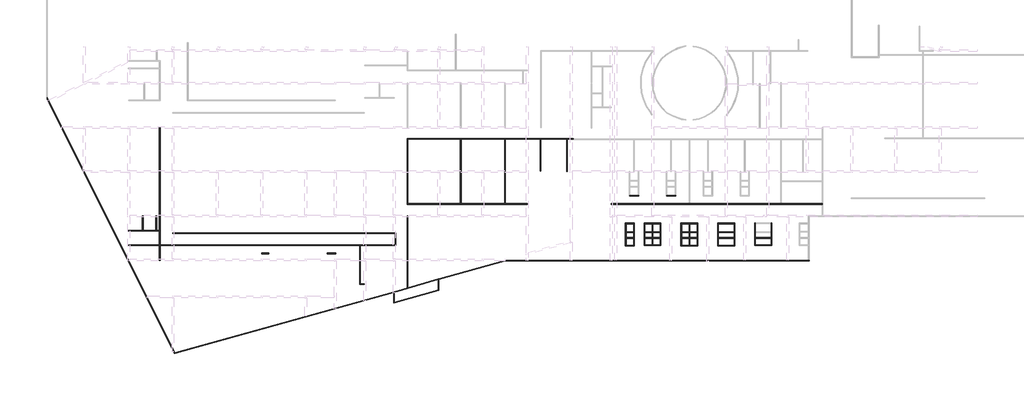
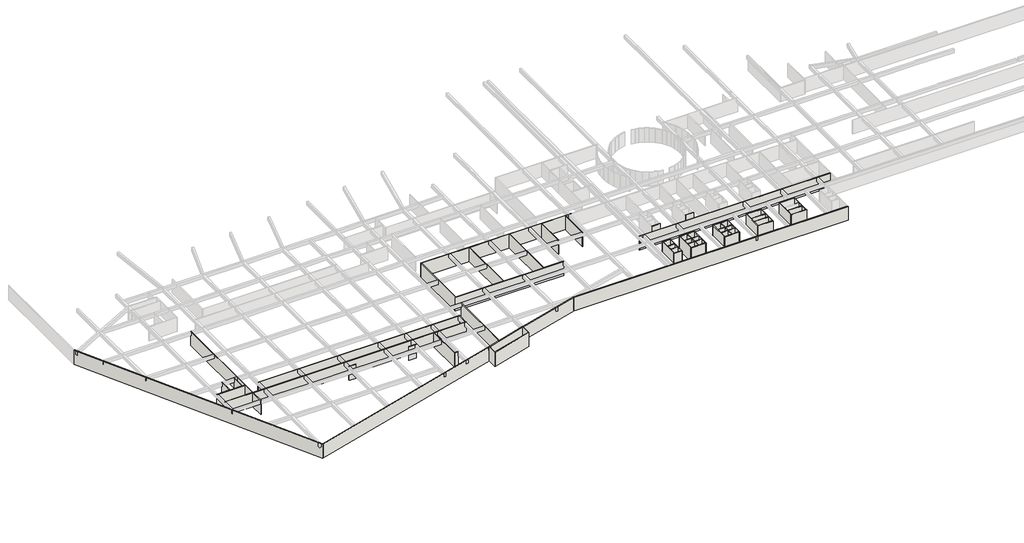
# One storey, part 1 of 8: 60 walls.
"""IFC4 building model written with IfcOpenShell, lengths in millimetres."""

from ifc_helpers import new_model, si_unit, origin, origin_with_axes, place, context, project, spatial, polyline, outline, extrude, faceted_brep, element, save

model = new_model("IFC4")

# Units and contexts
model_context = context("Model", 3, world=origin())
ifc_project = project(units=[si_unit("LENGTHUNIT", "METRE", prefix="MILLI")], contexts=[model_context])

# Site, building, storey
site = spatial("IfcSite", under=ifc_project)
building = spatial("IfcBuilding", under=site)
storey = spatial("IfcBuildingStorey", under=building, Name="户型图", Elevation=0.0)

# Walls
placement = place(None, origin())
element("IfcWall", 1, ObjectType="所有墙体", at=placement, inside=storey, context=model_context, shape_type="Brep", body=[
    faceted_brep([(299763.8653576, 3334.4623872, 0.0), (325653.4541666, -48444.7152378, 0.0), (325653.4541666, -48444.7152378, 3300.0), (299763.8653576, 3334.4623872, 3300.0), (299763.8653576, 3602.7905445, 0.0), (299763.8653576, 3602.7905445, 3300.0), (325716.5790893, -48302.6369258, 3300.0), (325771.2567723, -48411.9922918, 3300.0), (325771.2567723, -48411.9922918, 0.0), (325716.5790893, -48302.6369258, 0.0)], [[[0, 1, 2, 3]], [[4, 5, 6, 7, 8, 9]], [[1, 0, 4, 9, 8]], [[3, 2, 7, 6, 5]], [[0, 3, 5, 4]], [[2, 1, 8, 7]]]),
])
element("IfcWall", 2, ObjectType="所有墙体", at=placement, inside=storey, context=model_context, shape_type="Brep", body=[
    faceted_brep([(325771.2567723, -48411.9922918, 0.0), (370235.8958445, -36060.7036633, 0.0), (370355.8958445, -36027.37033, 0.0), (370355.8958445, -36027.37033, 3300.0), (370235.8958445, -36060.7036633, 3300.0), (325771.2567723, -48411.9922918, 3300.0), (325716.5790893, -48302.6369258, 0.0), (325716.5790893, -48302.6369258, 3300.0), (370355.8958445, -35902.8267187, 3300.0), (370355.8958445, -35902.8267187, 0.0), (370355.8958445, -36026.7458048, 0.0), (370355.8958445, -36026.7458048, 3300.0)], [[[0, 1, 2, 3, 4, 5]], [[6, 7, 8, 9]], [[2, 1, 0, 6, 9, 10]], [[5, 4, 3, 11, 8, 7]], [[0, 5, 7, 6]], [[3, 2, 10, 9, 8, 11]]]),
])
element("IfcWall", 3, ObjectType="所有墙体", at=placement, inside=storey, context=model_context, shape_type="Brep", body=[
    faceted_brep([(370235.8958445, -36060.7036633, 0.0), (370235.8958445, -38230.8455142, 0.0), (370235.8958445, -38230.8455142, 3300.0), (370235.8958445, -36060.7036633, 3300.0), (370355.8958445, -36027.37033, 0.0), (370355.8958445, -36027.37033, 3300.0), (370355.8958445, -38072.9685696, 3300.0), (370355.8958445, -38197.5121809, 3300.0), (370355.8958445, -38197.5121809, 0.0), (370355.8958445, -38072.9685696, 0.0)], [[[0, 1, 2, 3]], [[4, 5, 6, 7, 8, 9]], [[1, 0, 4, 9, 8]], [[3, 2, 7, 6, 5]], [[0, 3, 5, 4]], [[2, 1, 8, 7]]]),
])
element("IfcWall", 4, ObjectType="所有墙体", at=placement, inside=storey, context=model_context, shape_type="Brep", body=[
    faceted_brep([(370355.8958445, -38197.5121809, 0.0), (379412.9641952, -35681.6598618, 0.0), (379412.9641952, -35681.6598618, 3300.0), (370355.8958445, -38197.5121809, 3300.0), (370355.8958445, -38072.9685696, 0.0), (370355.8958445, -38072.9685696, 3300.0), (379292.9641952, -35590.4495838, 3300.0), (379412.9641952, -35557.1162505, 3300.0), (379412.9641952, -35557.1162505, 0.0), (379292.9641952, -35590.4495838, 0.0)], [[[0, 1, 2, 3]], [[4, 5, 6, 7, 8, 9]], [[1, 0, 4, 9, 8]], [[3, 2, 7, 6, 5]], [[0, 3, 5, 4]], [[2, 1, 8, 7]]]),
])
element("IfcWall", 5, ObjectType="所有墙体", at=placement, inside=storey, context=model_context, shape_type="Brep", body=[
    faceted_brep([(379412.9641952, -35557.1162505, 0.0), (379412.9641952, -33381.6598618, 0.0), (379412.9641952, -33257.1162505, 0.0), (379412.9641952, -33257.1162505, 3300.0), (379412.9641952, -33381.6598618, 3300.0), (379412.9641952, -35557.1162505, 3300.0), (379292.9641952, -35590.4495838, 0.0), (379292.9641952, -35590.4495838, 3300.0), (379292.9641952, -33416.0892021, 3300.0), (379292.9641952, -33291.074109, 3300.0), (379292.9641952, -33290.4495838, 3300.0), (379292.9641952, -33290.4495838, 0.0), (379292.9641952, -33291.074109, 0.0), (379292.9641952, -33416.0892021, 0.0)], [[[0, 1, 2, 3, 4, 5]], [[6, 7, 8, 9, 10, 11, 12, 13]], [[2, 1, 0, 6, 13, 12, 11]], [[5, 4, 3, 10, 9, 8, 7]], [[0, 5, 7, 6]], [[3, 2, 11, 10]]]),
])
element("IfcWall", 6, ObjectType="所有墙体", at=placement, inside=storey, context=model_context, shape_type="SweptSolid", body=[
    extrude(outline(polyline([(392926.9235644, -29627.78226), (379412.9641952, -33381.6598618), (379412.9641952, -33257.1162505), (392910.5665638, -29507.78226), (392926.9235644, -29627.78226)])), origin_with_axes(), (0.0, 0.0, 1.0), 3300.0),
])
element("IfcWall", 7, ObjectType="所有墙体", at=placement, inside=storey, context=model_context, shape_type="Brep", body=[
    faceted_brep([(392926.9235644, -29627.78226, 0.0), (454678.7450641, -29627.78226, 0.0), (454678.7450641, -29627.78226, 3300.0), (392926.9235644, -29627.78226, 3300.0), (392910.5665638, -29507.78226, 0.0), (392910.5665638, -29507.78226, 3300.0), (454558.7450641, -29507.78226, 3300.0), (454678.7450641, -29507.78226, 3300.0), (454678.7450641, -29507.78226, 0.0), (454558.7450641, -29507.78226, 0.0)], [[[0, 1, 2, 3]], [[4, 5, 6, 7, 8, 9]], [[1, 0, 4, 9, 8]], [[3, 2, 7, 6, 5]], [[0, 3, 5, 4]], [[2, 1, 8, 7]]]),
])
element("IfcWall", 8, ObjectType="所有墙体", at=placement, inside=storey, context=model_context, shape_type="Brep", body=[
    faceted_brep([(457393.8653576, -18001.3735105, 0.0), (449013.8653567, -18001.3735105, 0.0), (448893.8653567, -18001.3735105, 0.0), (430413.8653576, -18001.3735105, 0.0), (430293.8653576, -18001.3735105, 0.0), (414453.8653576, -18001.3735105, 0.0), (414453.8653576, -18001.3735105, 3300.0), (430293.8653576, -18001.3735105, 3300.0), (430413.8653576, -18001.3735105, 3300.0), (448893.8653567, -18001.3735105, 3300.0), (449013.8653567, -18001.3735105, 3300.0), (457393.8653576, -18001.3735105, 3300.0), (457393.8653576, -18121.3735105, 0.0), (457393.8653576, -18121.3735105, 3300.0), (414453.8653576, -18121.3735105, 3300.0), (414453.8653576, -18121.3735105, 0.0)], [[[0, 1, 2, 3, 4, 5, 6, 7, 8, 9, 10, 11]], [[12, 13, 14, 15]], [[5, 4, 3, 2, 1, 0, 12, 15]], [[6, 5, 15, 14]], [[11, 10, 9, 8, 7, 6, 14, 13]], [[0, 11, 13, 12]]]),
])
element("IfcWall", 9, ObjectType="所有墙体", at=placement, inside=storey, context=model_context, shape_type="Brep", body=[
    faceted_brep([(425763.8653576, -16421.3735096, 0.0), (427563.8653576, -16421.3735096, 0.0), (427563.8653576, -16421.3735096, 3300.0), (425763.8653576, -16421.3735096, 3300.0), (425763.8653576, -16301.3735096, 0.0), (425763.8653576, -16301.3735096, 3300.0), (427443.8653576, -16301.3735096, 3300.0), (427563.8653576, -16301.3735096, 3300.0), (427563.8653576, -16301.3735096, 0.0), (427443.8653576, -16301.3735096, 0.0)], [[[0, 1, 2, 3]], [[4, 5, 6, 7, 8, 9]], [[1, 0, 4, 9, 8]], [[3, 2, 7, 6, 5]], [[0, 3, 5, 4]], [[2, 1, 8, 7]]]),
])
element("IfcWall", 10, ObjectType="所有墙体", at=placement, inside=storey, context=model_context, shape_type="Brep", body=[
    faceted_brep([(418263.8653576, -16421.3261103, 0.0), (420063.8653576, -16421.3261103, 0.0), (420063.8653576, -16421.3261103, 3300.0), (418263.8653576, -16421.3261103, 3300.0), (418263.8653576, -16301.3261103, 0.0), (418263.8653576, -16301.3261103, 3300.0), (419943.8653576, -16301.3261103, 3300.0), (420063.8653576, -16301.3261103, 3300.0), (420063.8653576, -16301.3261103, 0.0), (419943.8653576, -16301.3261103, 0.0)], [[[0, 1, 2, 3]], [[4, 5, 6, 7, 8, 9]], [[1, 0, 4, 9, 8]], [[3, 2, 7, 6, 5]], [[0, 3, 5, 4]], [[2, 1, 8, 7]]]),
])
element("IfcWall", 11, ObjectType="所有墙体", at=placement, inside=storey, context=model_context, shape_type="Brep", body=[
    faceted_brep([(417343.8653576, -22071.3735096, 0.0), (417463.8653576, -22071.3735096, 0.0), (419043.8653576, -22071.3735096, 0.0), (419163.8653576, -22071.3735096, 0.0), (419163.8653576, -22071.3735096, 3300.0), (419043.8653576, -22071.3735096, 3300.0), (417463.8653576, -22071.3735096, 3300.0), (417343.8653576, -22071.3735096, 3300.0), (417343.8653576, -21951.3735096, 0.0), (417343.8653576, -21951.3735096, 3300.0), (419163.8653576, -21951.3735096, 3300.0), (419163.8653576, -21951.3735096, 0.0)], [[[0, 1, 2, 3, 4, 5, 6, 7]], [[8, 9, 10, 11]], [[3, 2, 1, 0, 8, 11]], [[7, 6, 5, 4, 10, 9]], [[4, 3, 11, 10]], [[0, 7, 9, 8]]]),
])
element("IfcWall", 12, ObjectType="所有墙体", at=placement, inside=storey, context=model_context, shape_type="Brep", body=[
    faceted_brep([(419043.8653576, -22071.3735096, 0.0), (419043.8653576, -23701.6182553, 0.0), (419043.8653576, -23821.6182553, 0.0), (419043.8653576, -24901.6891861, 0.0), (419043.8653576, -25021.6891861, 0.0), (419043.8653576, -26451.3735096, 0.0), (419043.8653576, -26571.3735096, 0.0), (419043.8653576, -26571.3735096, 3300.0), (419043.8653576, -26451.3735096, 3300.0), (419043.8653576, -25021.6891861, 3300.0), (419043.8653576, -24901.6891861, 3300.0), (419043.8653576, -23821.6182553, 3300.0), (419043.8653576, -23701.6182553, 3300.0), (419043.8653576, -22071.3735096, 3300.0), (419163.8653576, -22071.3735096, 0.0), (419163.8653576, -22071.3735096, 3300.0), (419163.8653576, -26571.3735096, 3300.0), (419163.8653576, -26571.3735096, 0.0)], [[[0, 1, 2, 3, 4, 5, 6, 7, 8, 9, 10, 11, 12, 13]], [[14, 15, 16, 17]], [[6, 5, 4, 3, 2, 1, 0, 14, 17]], [[13, 12, 11, 10, 9, 8, 7, 16, 15]], [[0, 13, 15, 14]], [[7, 6, 17, 16]]]),
])
element("IfcWall", 13, ObjectType="所有墙体", at=placement, inside=storey, context=model_context, shape_type="Brep", body=[
    faceted_brep([(419043.8653576, -26451.3735096, 0.0), (417463.8653576, -26451.3735096, 0.0), (417343.8653576, -26451.3735096, 0.0), (417343.8653576, -26451.3735096, 3300.0), (417463.8653576, -26451.3735096, 3300.0), (419043.8653576, -26451.3735096, 3300.0), (419043.8653576, -26571.3735096, 0.0), (419043.8653576, -26571.3735096, 3300.0), (417343.8653576, -26571.3735096, 3300.0), (417343.8653576, -26571.3735096, 0.0)], [[[0, 1, 2, 3, 4, 5]], [[6, 7, 8, 9]], [[2, 1, 0, 6, 9]], [[5, 4, 3, 8, 7]], [[0, 5, 7, 6]], [[3, 2, 9, 8]]]),
])
element("IfcWall", 14, ObjectType="所有墙体", at=placement, inside=storey, context=model_context, shape_type="Brep", body=[
    faceted_brep([(417463.8653576, -26451.3735096, 0.0), (417463.8653576, -25021.6891861, 0.0), (417463.8653576, -24901.6891861, 0.0), (417463.8653576, -23821.6182553, 0.0), (417463.8653576, -23701.6182553, 0.0), (417463.8653576, -22071.3735096, 0.0), (417463.8653576, -22071.3735096, 3300.0), (417463.8653576, -23701.6182553, 3300.0), (417463.8653576, -23821.6182553, 3300.0), (417463.8653576, -24901.6891861, 3300.0), (417463.8653576, -25021.6891861, 3300.0), (417463.8653576, -26451.3735096, 3300.0), (417343.8653576, -26451.3735096, 0.0), (417343.8653576, -26451.3735096, 3300.0), (417343.8653576, -22071.3735096, 3300.0), (417343.8653576, -22071.3735096, 0.0)], [[[0, 1, 2, 3, 4, 5, 6, 7, 8, 9, 10, 11]], [[12, 13, 14, 15]], [[5, 4, 3, 2, 1, 0, 12, 15]], [[11, 10, 9, 8, 7, 6, 14, 13]], [[6, 5, 15, 14]], [[0, 11, 13, 12]]]),
])
element("IfcWall", 15, ObjectType="所有墙体", at=placement, inside=storey, context=model_context, shape_type="SweptSolid", body=[
    extrude(outline(polyline([(417463.8653576, -23701.6182553), (419043.8653576, -23701.6182553), (419043.8653576, -23821.6182553), (417463.8653576, -23821.6182553), (417463.8653576, -23701.6182553)])), origin_with_axes(), (0.0, 0.0, 1.0), 3300.0),
])
element("IfcWall", 16, ObjectType="所有墙体", at=placement, inside=storey, context=model_context, shape_type="SweptSolid", body=[
    extrude(outline(polyline([(419043.8653576, -25021.6891861), (417463.8653576, -25021.6891861), (417463.8653576, -24901.6891861), (419043.8653576, -24901.6891861), (419043.8653576, -25021.6891861)])), origin_with_axes(), (0.0, 0.0, 1.0), 3300.0),
])
element("IfcWall", 17, ObjectType="所有墙体", at=placement, inside=storey, context=model_context, shape_type="Brep", body=[
    faceted_brep([(421144.3420584, -22071.3735096, 0.0), (421264.3420584, -22071.3735096, 0.0), (422793.8653536, -22071.3735096, 0.0), (422913.8653536, -22071.3735096, 0.0), (424443.3886489, -22071.3735096, 0.0), (424563.3886489, -22071.3735096, 0.0), (424563.3886489, -22071.3735096, 3300.0), (424443.3886489, -22071.3735096, 3300.0), (422913.8653536, -22071.3735096, 3300.0), (422793.8653536, -22071.3735096, 3300.0), (421264.3420584, -22071.3735096, 3300.0), (421144.3420584, -22071.3735096, 3300.0), (421144.3420584, -21951.3735096, 0.0), (421144.3420584, -21951.3735096, 3300.0), (424563.3886489, -21951.3735096, 3300.0), (424563.3886489, -21951.3735096, 0.0)], [[[0, 1, 2, 3, 4, 5, 6, 7, 8, 9, 10, 11]], [[12, 13, 14, 15]], [[5, 4, 3, 2, 1, 0, 12, 15]], [[11, 10, 9, 8, 7, 6, 14, 13]], [[6, 5, 15, 14]], [[0, 11, 13, 12]]]),
])
element("IfcWall", 18, ObjectType="所有墙体", at=placement, inside=storey, context=model_context, shape_type="Brep", body=[
    faceted_brep([(424443.3886489, -22071.3735096, 0.0), (424443.3886489, -23701.6182553, 0.0), (424443.3886489, -23821.6182553, 0.0), (424443.3886489, -24901.6891861, 0.0), (424443.3886489, -25021.6891861, 0.0), (424443.3886489, -26401.6891861, 0.0), (424443.3886489, -26521.6891861, 0.0), (424443.3886489, -26521.6891861, 3300.0), (424443.3886489, -26401.6891861, 3300.0), (424443.3886489, -25021.6891861, 3300.0), (424443.3886489, -24901.6891861, 3300.0), (424443.3886489, -23821.6182553, 3300.0), (424443.3886489, -23701.6182553, 3300.0), (424443.3886489, -22071.3735096, 3300.0), (424563.3886489, -22071.3735096, 0.0), (424563.3886489, -22071.3735096, 3300.0), (424563.3886489, -26521.6891861, 3300.0), (424563.3886489, -26521.6891861, 0.0)], [[[0, 1, 2, 3, 4, 5, 6, 7, 8, 9, 10, 11, 12, 13]], [[14, 15, 16, 17]], [[6, 5, 4, 3, 2, 1, 0, 14, 17]], [[13, 12, 11, 10, 9, 8, 7, 16, 15]], [[0, 13, 15, 14]], [[7, 6, 17, 16]]]),
])
element("IfcWall", 19, ObjectType="所有墙体", at=placement, inside=storey, context=model_context, shape_type="Brep", body=[
    faceted_brep([(424443.3886489, -26401.6891861, 0.0), (422913.8653536, -26401.6891861, 0.0), (422793.8653536, -26401.6891861, 0.0), (421264.3420584, -26401.6891861, 0.0), (421144.3420584, -26401.6891861, 0.0), (421144.3420584, -26401.6891861, 3300.0), (421264.3420584, -26401.6891861, 3300.0), (422793.8653536, -26401.6891861, 3300.0), (422913.8653536, -26401.6891861, 3300.0), (424443.3886489, -26401.6891861, 3300.0), (424443.3886489, -26521.6891861, 0.0), (424443.3886489, -26521.6891861, 3300.0), (421144.3420584, -26521.6891861, 3300.0), (421144.3420584, -26521.6891861, 0.0)], [[[0, 1, 2, 3, 4, 5, 6, 7, 8, 9]], [[10, 11, 12, 13]], [[4, 3, 2, 1, 0, 10, 13]], [[9, 8, 7, 6, 5, 12, 11]], [[0, 9, 11, 10]], [[5, 4, 13, 12]]]),
])
element("IfcWall", 20, ObjectType="所有墙体", at=placement, inside=storey, context=model_context, shape_type="Brep", body=[
    faceted_brep([(421264.3420584, -26401.6891861, 0.0), (421264.3420584, -25021.6891861, 0.0), (421264.3420584, -24901.6891861, 0.0), (421264.3420584, -23821.6182553, 0.0), (421264.3420584, -23701.6182553, 0.0), (421264.3420584, -22071.3735096, 0.0), (421264.3420584, -22071.3735096, 3300.0), (421264.3420584, -23701.6182553, 3300.0), (421264.3420584, -23821.6182553, 3300.0), (421264.3420584, -24901.6891861, 3300.0), (421264.3420584, -25021.6891861, 3300.0), (421264.3420584, -26401.6891861, 3300.0), (421144.3420584, -26401.6891861, 0.0), (421144.3420584, -26401.6891861, 3300.0), (421144.3420584, -22071.3735096, 3300.0), (421144.3420584, -22071.3735096, 0.0)], [[[0, 1, 2, 3, 4, 5, 6, 7, 8, 9, 10, 11]], [[12, 13, 14, 15]], [[5, 4, 3, 2, 1, 0, 12, 15]], [[11, 10, 9, 8, 7, 6, 14, 13]], [[0, 11, 13, 12]], [[6, 5, 15, 14]]]),
])
element("IfcWall", 21, ObjectType="所有墙体", at=placement, inside=storey, context=model_context, shape_type="Brep", body=[
    faceted_brep([(422793.8653536, -22071.3735096, 0.0), (422793.8653536, -23701.6182553, 0.0), (422793.8653536, -23821.6182553, 0.0), (422793.8653536, -24901.6891861, 0.0), (422793.8653536, -25021.6891861, 0.0), (422793.8653536, -26401.6891861, 0.0), (422793.8653536, -26401.6891861, 3300.0), (422793.8653536, -25021.6891861, 3300.0), (422793.8653536, -24901.6891861, 3300.0), (422793.8653536, -23821.6182553, 3300.0), (422793.8653536, -23701.6182553, 3300.0), (422793.8653536, -22071.3735096, 3300.0), (422913.8653536, -22071.3735096, 0.0), (422913.8653536, -22071.3735096, 3300.0), (422913.8653536, -23701.6182553, 3300.0), (422913.8653536, -23821.6182553, 3300.0), (422913.8653536, -24901.6891861, 3300.0), (422913.8653536, -25021.6891861, 3300.0), (422913.8653536, -26401.6891861, 3300.0), (422913.8653536, -26401.6891861, 0.0), (422913.8653536, -25021.6891861, 0.0), (422913.8653536, -24901.6891861, 0.0), (422913.8653536, -23821.6182553, 0.0), (422913.8653536, -23701.6182553, 0.0)], [[[0, 1, 2, 3, 4, 5, 6, 7, 8, 9, 10, 11]], [[12, 13, 14, 15, 16, 17, 18, 19, 20, 21, 22, 23]], [[5, 4, 3, 2, 1, 0, 12, 23, 22, 21, 20, 19]], [[11, 10, 9, 8, 7, 6, 18, 17, 16, 15, 14, 13]], [[0, 11, 13, 12]], [[6, 5, 19, 18]]]),
])
element("IfcWall", 22, ObjectType="所有墙体", at=placement, inside=storey, context=model_context, shape_type="SweptSolid", body=[
    extrude(outline(polyline([(424443.3886489, -23701.6182553), (424443.3886489, -23821.6182553), (422913.8653536, -23821.6182553), (422913.8653536, -23701.6182553), (424443.3886489, -23701.6182553)])), origin_with_axes(), (0.0, 0.0, 1.0), 3300.0),
    extrude(outline(polyline([(421264.3420584, -23821.6182553), (421264.3420584, -23701.6182553), (422793.8653536, -23701.6182553), (422793.8653536, -23821.6182553), (421264.3420584, -23821.6182553)])), origin_with_axes(), (0.0, 0.0, 1.0), 3300.0),
])
element("IfcWall", 23, ObjectType="所有墙体", at=placement, inside=storey, context=model_context, shape_type="SweptSolid", body=[
    extrude(outline(polyline([(424443.3886489, -24901.6891861), (424443.3886489, -25021.6891861), (422913.8653536, -25021.6891861), (422913.8653536, -24901.6891861), (424443.3886489, -24901.6891861)])), origin_with_axes(), (0.0, 0.0, 1.0), 3300.0),
    extrude(outline(polyline([(421264.3420584, -25021.6891861), (421264.3420584, -24901.6891861), (422793.8653536, -24901.6891861), (422793.8653536, -25021.6891861), (421264.3420584, -25021.6891861)])), origin_with_axes(), (0.0, 0.0, 1.0), 3300.0),
])
element("IfcWall", 24, ObjectType="所有墙体", at=placement, inside=storey, context=model_context, shape_type="Brep", body=[
    faceted_brep([(428643.3886489, -22071.3735096, 0.0), (428763.3886489, -22071.3735096, 0.0), (430293.3886489, -22071.3735096, 0.0), (430413.3886489, -22071.3735096, 0.0), (431943.3886489, -22071.3735096, 0.0), (432063.3886489, -22071.3735096, 0.0), (432063.3886489, -22071.3735096, 3300.0), (431943.3886489, -22071.3735096, 3300.0), (430413.3886489, -22071.3735096, 3300.0), (430293.3886489, -22071.3735096, 3300.0), (428763.3886489, -22071.3735096, 3300.0), (428643.3886489, -22071.3735096, 3300.0), (428643.3886489, -21951.3735096, 0.0), (428643.3886489, -21951.3735096, 3300.0), (432063.3886489, -21951.3735096, 3300.0), (432063.3886489, -21951.3735096, 0.0)], [[[0, 1, 2, 3, 4, 5, 6, 7, 8, 9, 10, 11]], [[12, 13, 14, 15]], [[5, 4, 3, 2, 1, 0, 12, 15]], [[11, 10, 9, 8, 7, 6, 14, 13]], [[6, 5, 15, 14]], [[0, 11, 13, 12]]]),
])
element("IfcWall", 25, ObjectType="所有墙体", at=placement, inside=storey, context=model_context, shape_type="Brep", body=[
    faceted_brep([(431943.3886489, -22071.3735096, 0.0), (431943.3886489, -23701.6182553, 0.0), (431943.3886489, -23821.6182553, 0.0), (431943.3886489, -24901.6891861, 0.0), (431943.3886489, -25021.6891861, 0.0), (431943.3886489, -26451.6891861, 0.0), (431943.3886489, -26571.6891861, 0.0), (431943.3886489, -26571.6891861, 3300.0), (431943.3886489, -26451.6891861, 3300.0), (431943.3886489, -25021.6891861, 3300.0), (431943.3886489, -24901.6891861, 3300.0), (431943.3886489, -23821.6182553, 3300.0), (431943.3886489, -23701.6182553, 3300.0), (431943.3886489, -22071.3735096, 3300.0), (432063.3886489, -22071.3735096, 0.0), (432063.3886489, -22071.3735096, 3300.0), (432063.3886489, -26571.6891861, 3300.0), (432063.3886489, -26571.6891861, 0.0)], [[[0, 1, 2, 3, 4, 5, 6, 7, 8, 9, 10, 11, 12, 13]], [[14, 15, 16, 17]], [[6, 5, 4, 3, 2, 1, 0, 14, 17]], [[13, 12, 11, 10, 9, 8, 7, 16, 15]], [[0, 13, 15, 14]], [[7, 6, 17, 16]]]),
])
element("IfcWall", 26, ObjectType="所有墙体", at=placement, inside=storey, context=model_context, shape_type="Brep", body=[
    faceted_brep([(431943.3886489, -26451.6891861, 0.0), (430413.3886489, -26451.6891861, 0.0), (430293.3886489, -26451.6891861, 0.0), (428763.3886489, -26451.6891861, 0.0), (428643.3886489, -26451.6891861, 0.0), (428643.3886489, -26451.6891861, 3300.0), (428763.3886489, -26451.6891861, 3300.0), (430293.3886489, -26451.6891861, 3300.0), (430413.3886489, -26451.6891861, 3300.0), (431943.3886489, -26451.6891861, 3300.0), (431943.3886489, -26571.6891861, 0.0), (431943.3886489, -26571.6891861, 3300.0), (428643.3886489, -26571.6891861, 3300.0), (428643.3886489, -26571.6891861, 0.0)], [[[0, 1, 2, 3, 4, 5, 6, 7, 8, 9]], [[10, 11, 12, 13]], [[4, 3, 2, 1, 0, 10, 13]], [[9, 8, 7, 6, 5, 12, 11]], [[0, 9, 11, 10]], [[5, 4, 13, 12]]]),
])
element("IfcWall", 27, ObjectType="所有墙体", at=placement, inside=storey, context=model_context, shape_type="Brep", body=[
    faceted_brep([(428763.3886489, -26451.6891861, 0.0), (428763.3886489, -25021.6891861, 0.0), (428763.3886489, -24901.6891861, 0.0), (428763.3886489, -23821.6182553, 0.0), (428763.3886489, -23701.6182553, 0.0), (428763.3886489, -22071.3735096, 0.0), (428763.3886489, -22071.3735096, 3300.0), (428763.3886489, -23701.6182553, 3300.0), (428763.3886489, -23821.6182553, 3300.0), (428763.3886489, -24901.6891861, 3300.0), (428763.3886489, -25021.6891861, 3300.0), (428763.3886489, -26451.6891861, 3300.0), (428643.3886489, -26451.6891861, 0.0), (428643.3886489, -26451.6891861, 3300.0), (428643.3886489, -22071.3735096, 3300.0), (428643.3886489, -22071.3735096, 0.0)], [[[0, 1, 2, 3, 4, 5, 6, 7, 8, 9, 10, 11]], [[12, 13, 14, 15]], [[5, 4, 3, 2, 1, 0, 12, 15]], [[11, 10, 9, 8, 7, 6, 14, 13]], [[6, 5, 15, 14]], [[0, 11, 13, 12]]]),
])
element("IfcWall", 28, ObjectType="所有墙体", at=placement, inside=storey, context=model_context, shape_type="Brep", body=[
    faceted_brep([(428763.3886489, -23821.6182553, 0.0), (430293.3886489, -23821.6182553, 0.0), (430413.3886489, -23821.6182553, 0.0), (431943.3886489, -23821.6182553, 0.0), (431943.3886489, -23821.6182553, 3300.0), (430413.3886489, -23821.6182553, 3300.0), (430293.3886489, -23821.6182553, 3300.0), (428763.3886489, -23821.6182553, 3300.0), (428763.3886489, -23701.6182553, 0.0), (428763.3886489, -23701.6182553, 3300.0), (430293.3886489, -23701.6182553, 3300.0), (430413.3886489, -23701.6182553, 3300.0), (431943.3886489, -23701.6182553, 3300.0), (431943.3886489, -23701.6182553, 0.0), (430413.3886489, -23701.6182553, 0.0), (430293.3886489, -23701.6182553, 0.0)], [[[0, 1, 2, 3, 4, 5, 6, 7]], [[8, 9, 10, 11, 12, 13, 14, 15]], [[3, 2, 1, 0, 8, 15, 14, 13]], [[7, 6, 5, 4, 12, 11, 10, 9]], [[4, 3, 13, 12]], [[0, 7, 9, 8]]]),
])
element("IfcWall", 29, ObjectType="所有墙体", at=placement, inside=storey, context=model_context, shape_type="Brep", body=[
    faceted_brep([(431943.3886489, -24901.6891861, 0.0), (430413.3886489, -24901.6891861, 0.0), (430293.3886489, -24901.6891861, 0.0), (428763.3886489, -24901.6891861, 0.0), (428763.3886489, -24901.6891861, 3300.0), (430293.3886489, -24901.6891861, 3300.0), (430413.3886489, -24901.6891861, 3300.0), (431943.3886489, -24901.6891861, 3300.0), (431943.3886489, -25021.6891861, 0.0), (431943.3886489, -25021.6891861, 3300.0), (430413.3886489, -25021.6891861, 3300.0), (430293.3886489, -25021.6891861, 3300.0), (428763.3886489, -25021.6891861, 3300.0), (428763.3886489, -25021.6891861, 0.0), (430293.3886489, -25021.6891861, 0.0), (430413.3886489, -25021.6891861, 0.0)], [[[0, 1, 2, 3, 4, 5, 6, 7]], [[8, 9, 10, 11, 12, 13, 14, 15]], [[3, 2, 1, 0, 8, 15, 14, 13]], [[7, 6, 5, 4, 12, 11, 10, 9]], [[0, 7, 9, 8]], [[4, 3, 13, 12]]]),
])
element("IfcWall", 30, ObjectType="所有墙体", at=placement, inside=storey, context=model_context, shape_type="SweptSolid", body=[
    extrude(outline(polyline([(430293.3886489, -22071.3735096), (430413.3886489, -22071.3735096), (430413.3886489, -23701.6182553), (430293.3886489, -23701.6182553), (430293.3886489, -22071.3735096)])), origin_with_axes(), (0.0, 0.0, 1.0), 3300.0),
    extrude(outline(polyline([(430413.3886489, -26451.6891861), (430293.3886489, -26451.6891861), (430293.3886489, -25021.6891861), (430413.3886489, -25021.6891861), (430413.3886489, -26451.6891861)])), origin_with_axes(), (0.0, 0.0, 1.0), 3300.0),
    extrude(outline(polyline([(430293.3886489, -23821.6182553), (430413.3886489, -23821.6182553), (430413.3886489, -24901.6891861), (430293.3886489, -24901.6891861), (430293.3886489, -23821.6182553)])), origin_with_axes(), (0.0, 0.0, 1.0), 3300.0),
])
element("IfcWall", 31, ObjectType="所有墙体", at=placement, inside=storey, context=model_context, shape_type="Brep", body=[
    faceted_brep([(436144.3420663, -21951.6891861, 0.0), (436144.3420663, -26571.6891861, 0.0), (436144.3420663, -26571.6891861, 3300.0), (436144.3420663, -21951.6891861, 3300.0), (436264.3420663, -21951.6891861, 0.0), (436264.3420663, -21951.6891861, 3300.0), (436264.3420663, -22071.6891861, 3300.0), (436264.3420663, -23701.6182553, 3300.0), (436264.3420663, -23821.6182553, 3300.0), (436264.3420663, -24901.6891861, 3300.0), (436264.3420663, -25021.6891861, 3300.0), (436264.3420663, -26451.6891861, 3300.0), (436264.3420663, -26571.6891861, 3300.0), (436264.3420663, -26571.6891861, 0.0), (436264.3420663, -26451.6891861, 0.0), (436264.3420663, -25021.6891861, 0.0), (436264.3420663, -24901.6891861, 0.0), (436264.3420663, -23821.6182553, 0.0), (436264.3420663, -23701.6182553, 0.0), (436264.3420663, -22071.6891861, 0.0)], [[[0, 1, 2, 3]], [[4, 5, 6, 7, 8, 9, 10, 11, 12, 13, 14, 15, 16, 17, 18, 19]], [[1, 0, 4, 19, 18, 17, 16, 15, 14, 13]], [[3, 2, 12, 11, 10, 9, 8, 7, 6, 5]], [[2, 1, 13, 12]], [[0, 3, 5, 4]]]),
])
element("IfcWall", 32, ObjectType="所有墙体", at=placement, inside=storey, context=model_context, shape_type="Brep", body=[
    faceted_brep([(436264.3420663, -26571.6891861, 0.0), (439564.3420663, -26571.6891861, 0.0), (439564.3420663, -26571.6891861, 3300.0), (436264.3420663, -26571.6891861, 3300.0), (436264.3420663, -26451.6891861, 0.0), (436264.3420663, -26451.6891861, 3300.0), (439444.3420663, -26451.6891861, 3300.0), (439564.3420663, -26451.6891861, 3300.0), (439564.3420663, -26451.6891861, 0.0), (439444.3420663, -26451.6891861, 0.0)], [[[0, 1, 2, 3]], [[4, 5, 6, 7, 8, 9]], [[1, 0, 4, 9, 8]], [[3, 2, 7, 6, 5]], [[0, 3, 5, 4]], [[2, 1, 8, 7]]]),
])
element("IfcWall", 33, ObjectType="所有墙体", at=placement, inside=storey, context=model_context, shape_type="Brep", body=[
    faceted_brep([(439564.3420663, -26451.6891861, 0.0), (439564.3420663, -21951.6891861, 0.0), (439564.3420663, -21951.6891861, 3300.0), (439564.3420663, -26451.6891861, 3300.0), (439444.3420663, -26451.6891861, 0.0), (439444.3420663, -26451.6891861, 3300.0), (439444.3420663, -25021.6891861, 3300.0), (439444.3420663, -24901.6891861, 3300.0), (439444.3420663, -23821.6182553, 3300.0), (439444.3420663, -23701.6182553, 3300.0), (439444.3420663, -22071.6891861, 3300.0), (439444.3420663, -21951.6891861, 3300.0), (439444.3420663, -21951.6891861, 0.0), (439444.3420663, -22071.6891861, 0.0), (439444.3420663, -23701.6182553, 0.0), (439444.3420663, -23821.6182553, 0.0), (439444.3420663, -24901.6891861, 0.0), (439444.3420663, -25021.6891861, 0.0)], [[[0, 1, 2, 3]], [[4, 5, 6, 7, 8, 9, 10, 11, 12, 13, 14, 15, 16, 17]], [[1, 0, 4, 17, 16, 15, 14, 13, 12]], [[3, 2, 11, 10, 9, 8, 7, 6, 5]], [[0, 3, 5, 4]], [[2, 1, 12, 11]]]),
])
element("IfcWall", 34, ObjectType="所有墙体", at=placement, inside=storey, context=model_context, shape_type="SweptSolid", body=[
    extrude(outline(polyline([(436264.3420663, -21951.6891861), (439444.3420663, -21951.6891861), (439444.3420663, -22071.6891861), (436264.3420663, -22071.6891861), (436264.3420663, -21951.6891861)])), origin_with_axes(), (0.0, 0.0, 1.0), 3300.0),
])
element("IfcWall", 35, ObjectType="所有墙体", at=placement, inside=storey, context=model_context, shape_type="SweptSolid", body=[
    extrude(outline(polyline([(439444.3420663, -23821.6182553), (436264.3420663, -23821.6182553), (436264.3420663, -23701.6182553), (439444.3420663, -23701.6182553), (439444.3420663, -23821.6182553)])), origin_with_axes(), (0.0, 0.0, 1.0), 3300.0),
])
element("IfcWall", 36, ObjectType="所有墙体", at=placement, inside=storey, context=model_context, shape_type="SweptSolid", body=[
    extrude(outline(polyline([(436264.3420663, -24901.6891861), (439444.3420663, -24901.6891861), (439444.3420663, -25021.6891861), (436264.3420663, -25021.6891861), (436264.3420663, -24901.6891861)])), origin_with_axes(), (0.0, 0.0, 1.0), 3300.0),
])
element("IfcWall", 37, ObjectType="所有墙体", at=placement, inside=storey, context=model_context, shape_type="Brep", body=[
    faceted_brep([(443593.8653655, -21921.3735096, 0.0), (443593.8653655, -26521.3735096, 0.0), (443593.8653655, -26521.3735096, 3300.0), (443593.8653655, -21921.3735096, 3300.0), (443713.8653655, -21921.3735096, 0.0), (443713.8653655, -21921.3735096, 3300.0), (443713.8653655, -22041.3735096, 3300.0), (443713.8653655, -23701.6182553, 3300.0), (443713.8653655, -23821.6182553, 3300.0), (443713.8653655, -24901.6891611, 3300.0), (443713.8653655, -25021.6891611, 3300.0), (443713.8653655, -26401.3735096, 3300.0), (443713.8653655, -26521.3735096, 3300.0), (443713.8653655, -26521.3735096, 0.0), (443713.8653655, -26401.3735096, 0.0), (443713.8653655, -25021.6891611, 0.0), (443713.8653655, -24901.6891611, 0.0), (443713.8653655, -23821.6182553, 0.0), (443713.8653655, -23701.6182553, 0.0), (443713.8653655, -22041.3735096, 0.0)], [[[0, 1, 2, 3]], [[4, 5, 6, 7, 8, 9, 10, 11, 12, 13, 14, 15, 16, 17, 18, 19]], [[1, 0, 4, 19, 18, 17, 16, 15, 14, 13]], [[3, 2, 12, 11, 10, 9, 8, 7, 6, 5]], [[2, 1, 13, 12]], [[0, 3, 5, 4]]]),
])
element("IfcWall", 38, ObjectType="所有墙体", at=placement, inside=storey, context=model_context, shape_type="Brep", body=[
    faceted_brep([(443713.8653655, -26521.3735096, 0.0), (447113.8653655, -26521.3735096, 0.0), (447113.8653655, -26521.3735096, 3300.0), (443713.8653655, -26521.3735096, 3300.0), (443713.8653655, -26401.3735096, 0.0), (443713.8653655, -26401.3735096, 3300.0), (446993.8653655, -26401.3735096, 3300.0), (447113.8653655, -26401.3735096, 3300.0), (447113.8653655, -26401.3735096, 0.0), (446993.8653655, -26401.3735096, 0.0)], [[[0, 1, 2, 3]], [[4, 5, 6, 7, 8, 9]], [[1, 0, 4, 9, 8]], [[3, 2, 7, 6, 5]], [[0, 3, 5, 4]], [[2, 1, 8, 7]]]),
])
element("IfcWall", 39, ObjectType="所有墙体", at=placement, inside=storey, context=model_context, shape_type="Brep", body=[
    faceted_brep([(447113.8653655, -26401.3735096, 0.0), (447113.8653655, -21921.3735096, 0.0), (447113.8653655, -21921.3735096, 3300.0), (447113.8653655, -26401.3735096, 3300.0), (446993.8653655, -26401.3735096, 0.0), (446993.8653655, -26401.3735096, 3300.0), (446993.8653655, -25021.6891611, 3300.0), (446993.8653655, -24901.6891611, 3300.0), (446993.8653655, -23821.6182553, 3300.0), (446993.8653655, -23701.6182553, 3300.0), (446993.8653655, -22041.3735096, 3300.0), (446993.8653655, -21921.3735096, 3300.0), (446993.8653655, -21921.3735096, 0.0), (446993.8653655, -22041.3735096, 0.0), (446993.8653655, -23701.6182553, 0.0), (446993.8653655, -23821.6182553, 0.0), (446993.8653655, -24901.6891611, 0.0), (446993.8653655, -25021.6891611, 0.0)], [[[0, 1, 2, 3]], [[4, 5, 6, 7, 8, 9, 10, 11, 12, 13, 14, 15, 16, 17]], [[1, 0, 4, 17, 16, 15, 14, 13, 12]], [[3, 2, 11, 10, 9, 8, 7, 6, 5]], [[0, 3, 5, 4]], [[2, 1, 12, 11]]]),
])
element("IfcWall", 40, ObjectType="所有墙体", at=placement, inside=storey, context=model_context, shape_type="SweptSolid", body=[
    extrude(outline(polyline([(443713.8653655, -24901.6891611), (446993.8653655, -24901.6891611), (446993.8653655, -25021.6891611), (443713.8653655, -25021.6891611), (443713.8653655, -24901.6891611)])), origin_with_axes(), (0.0, 0.0, 1.0), 3300.0),
])
element("IfcWall", 41, ObjectType="所有墙体", at=placement, inside=storey, context=model_context, shape_type="Brep", body=[
    faceted_brep([(322593.8653576, -2461.3735096, 0.0), (322593.8653576, -23451.3735136, 0.0), (322593.8653576, -23571.3735136, 0.0), (322593.8653576, -26401.3735096, 0.0), (322593.8653576, -26521.3735096, 0.0), (322593.8653576, -29575.9633131, 0.0), (322593.8653576, -29575.9633131, 3300.0), (322593.8653576, -26521.3735096, 3300.0), (322593.8653576, -26401.3735096, 3300.0), (322593.8653576, -23571.3735136, 3300.0), (322593.8653576, -23451.3735136, 3300.0), (322593.8653576, -2461.3735096, 3300.0), (322713.8653576, -2461.3735096, 0.0), (322713.8653576, -2461.3735096, 3300.0), (322713.8653576, -26401.3735096, 3300.0), (322713.8653576, -26521.3735096, 3300.0), (322713.8653576, -29575.9633131, 3300.0), (322713.8653576, -29575.9633131, 0.0), (322713.8653576, -26521.3735096, 0.0), (322713.8653576, -26401.3735096, 0.0)], [[[0, 1, 2, 3, 4, 5, 6, 7, 8, 9, 10, 11]], [[12, 13, 14, 15, 16, 17, 18, 19]], [[5, 4, 3, 2, 1, 0, 12, 19, 18, 17]], [[6, 5, 17, 16]], [[11, 10, 9, 8, 7, 6, 16, 15, 14, 13]], [[0, 11, 13, 12]]]),
])
element("IfcWall", 42, ObjectType="所有墙体", at=placement, inside=storey, context=model_context, shape_type="Brep", body=[
    faceted_brep([(316353.8653576, -26521.3735096, 3300.0), (316353.8653576, -26521.3735096, 0.0), (322593.8653576, -26521.3735096, 0.0), (322593.8653576, -26521.3735096, 3300.0), (316353.8653576, -26401.3735096, 0.0), (316353.8653576, -26401.3735096, 3300.0), (322593.8653576, -26401.3735096, 3300.0), (322593.8653576, -26401.3735096, 0.0)], [[[0, 1, 2, 3]], [[4, 5, 6, 7]], [[1, 4, 7, 2]], [[5, 0, 3, 6]], [[1, 0, 5, 4]], [[3, 2, 7, 6]]]),
    faceted_brep([(370613.8653576, -26521.3735096, 0.0), (370613.8653576, -26521.3735096, 3300.0), (363413.8653576, -26521.3735096, 3300.0), (363293.8653576, -26521.3735096, 3300.0), (322713.8653576, -26521.3735096, 3300.0), (322713.8653576, -26521.3735096, 0.0), (363293.8653576, -26521.3735096, 0.0), (363413.8653576, -26521.3735096, 0.0), (370613.8653576, -26401.3735096, 3300.0), (370613.8653576, -26401.3735096, 0.0), (370493.8653576, -26401.3735096, 0.0), (322713.8653576, -26401.3735096, 0.0), (322713.8653576, -26401.3735096, 3300.0), (370493.8653576, -26401.3735096, 3300.0)], [[[0, 1, 2, 3, 4, 5, 6, 7]], [[8, 9, 10, 11, 12, 13]], [[9, 0, 7, 6, 5, 11, 10]], [[1, 8, 13, 12, 4, 3, 2]], [[5, 4, 12, 11]], [[1, 0, 9, 8]]]),
])
element("IfcWall", 43, ObjectType="所有墙体", at=placement, inside=storey, context=model_context, shape_type="Brep", body=[
    faceted_brep([(370613.8653576, -26401.3735096, 0.0), (370613.8653576, -23901.3735066, 0.0), (370613.8653576, -23901.3735066, 3300.0), (370613.8653576, -26401.3735096, 3300.0), (370493.8653576, -26401.3735096, 0.0), (370493.8653576, -26401.3735096, 3300.0), (370493.8653576, -24021.3735066, 3300.0), (370493.8653576, -23901.3735066, 3300.0), (370493.8653576, -23901.3735066, 0.0), (370493.8653576, -24021.3735066, 0.0)], [[[0, 1, 2, 3]], [[4, 5, 6, 7, 8, 9]], [[1, 0, 4, 9, 8]], [[3, 2, 7, 6, 5]], [[0, 3, 5, 4]], [[2, 1, 8, 7]]]),
])
element("IfcWall", 44, ObjectType="所有墙体", at=placement, inside=storey, context=model_context, shape_type="SweptSolid", body=[
    extrude(outline(polyline([(325253.8653576, -23901.3735066), (370493.8653576, -23901.3735066), (370493.8653576, -24021.3735066), (325253.8653576, -24021.3735066), (325253.8653576, -23901.3735066)])), origin_with_axes(), (0.0, 0.0, 1.0), 3300.0),
])
element("IfcWall", 45, ObjectType="所有墙体", at=placement, inside=storey, context=model_context, shape_type="Brep", body=[
    faceted_brep([(316253.8653575, -23571.3735136, 0.0), (322593.8653576, -23571.3735136, 0.0), (322593.8653576, -23571.3735136, 3300.0), (316253.8653575, -23571.3735136, 3300.0), (316253.8653575, -23451.3735136, 0.0), (316253.8653575, -23451.3735136, 3300.0), (319143.8653576, -23451.3735136, 3300.0), (319263.8653576, -23451.3735136, 3300.0), (321893.8653576, -23451.3735136, 3300.0), (322013.8653576, -23451.3735136, 3300.0), (322593.8653576, -23451.3735136, 3300.0), (322593.8653576, -23451.3735136, 0.0), (322013.8653576, -23451.3735136, 0.0), (321893.8653576, -23451.3735136, 0.0), (319263.8653576, -23451.3735136, 0.0), (319143.8653576, -23451.3735136, 0.0)], [[[0, 1, 2, 3]], [[4, 5, 6, 7, 8, 9, 10, 11, 12, 13, 14, 15]], [[1, 0, 4, 15, 14, 13, 12, 11]], [[3, 2, 10, 9, 8, 7, 6, 5]], [[0, 3, 5, 4]], [[2, 1, 11, 10]]]),
])
element("IfcWall", 46, ObjectType="所有墙体", at=placement, inside=storey, context=model_context, shape_type="SweptSolid", body=[
    extrude(outline(polyline([(319143.8653576, -23451.3735136), (319143.8653576, -20461.3735096), (319263.8653576, -20461.3735096), (319263.8653576, -23451.3735136), (319143.8653576, -23451.3735136)])), origin_with_axes(), (0.0, 0.0, 1.0), 3300.0),
])
element("IfcWall", 47, ObjectType="所有墙体", at=placement, inside=storey, context=model_context, shape_type="SweptSolid", body=[
    extrude(outline(polyline([(321893.8653576, -23451.3735136), (321893.8653576, -20461.3735096), (322013.8653576, -20461.3735096), (322013.8653576, -23451.3735136), (321893.8653576, -23451.3735136)])), origin_with_axes(), (0.0, 0.0, 1.0), 3300.0),
])
element("IfcWall", 48, ObjectType="所有墙体", at=placement, inside=storey, context=model_context, shape_type="SweptSolid", body=[
    extrude(outline(polyline([(344853.8653576, -28171.3735203), (343353.8653576, -28171.3735203), (343353.8653576, -28051.3735203), (344853.8653576, -28051.3735203), (344853.8653576, -28171.3735203)])), origin_with_axes(), (0.0, 0.0, 1.0), 3300.0),
])
element("IfcWall", 49, ObjectType="所有墙体", at=placement, inside=storey, context=model_context, shape_type="SweptSolid", body=[
    extrude(outline(polyline([(356753.8653576, -28051.3735204), (358453.8653576, -28051.3735204), (358453.8653576, -28171.3735204), (356753.8653576, -28171.3735204), (356753.8653576, -28051.3735204)])), origin_with_axes(), (0.0, 0.0, 1.0), 3300.0),
])
element("IfcWall", 50, ObjectType="所有墙体", at=placement, inside=storey, context=model_context, shape_type="Brep", body=[
    faceted_brep([(363293.8653576, -26521.3735096, 0.0), (363293.8653576, -34421.37351, 0.0), (363293.8653576, -34421.37351, 3300.0), (363293.8653576, -26521.3735096, 3300.0), (363413.8653576, -26521.3735096, 0.0), (363413.8653576, -26521.3735096, 3300.0), (363413.8653576, -34301.37351, 3300.0), (363413.8653576, -34421.37351, 3300.0), (363413.8653576, -34421.37351, 0.0), (363413.8653576, -34301.37351, 0.0)], [[[0, 1, 2, 3]], [[4, 5, 6, 7, 8, 9]], [[1, 0, 4, 9, 8]], [[3, 2, 7, 6, 5]], [[0, 3, 5, 4]], [[2, 1, 8, 7]]]),
])
element("IfcWall", 51, ObjectType="所有墙体", at=placement, inside=storey, context=model_context, shape_type="SweptSolid", body=[
    extrude(outline(polyline([(364253.8653576, -34421.37351), (363413.8653576, -34421.37351), (363413.8653576, -34301.37351), (364253.8653576, -34301.37351), (364253.8653576, -34421.37351)])), origin_with_axes(), (0.0, 0.0, 1.0), 3300.0),
])
element("IfcWall", 52, ObjectType="所有墙体", at=placement, inside=storey, context=model_context, shape_type="Brep", body=[
    faceted_brep([(370355.8958445, -36026.7458048, 0.0), (379292.9641952, -33416.0892021, 0.0), (379292.9641952, -33416.0892021, 3300.0), (370355.8958445, -36026.7458048, 3300.0), (370355.8958445, -35901.7307117, 0.0), (370355.8958445, -35901.7307117, 3300.0), (372993.8653577, -35131.1388065, 3300.0), (373113.8653577, -35096.084941, 3300.0), (379292.9641952, -33291.074109, 3300.0), (379292.9641952, -33291.074109, 0.0), (373113.8653577, -35096.084941, 0.0), (372993.8653577, -35131.1388065, 0.0), (370355.8958445, -35902.8267187, 0.0), (370355.8958445, -35902.8267187, 3300.0)], [[[0, 1, 2, 3]], [[4, 5, 6, 7, 8, 9, 10, 11]], [[1, 0, 12, 4, 11, 10, 9]], [[3, 2, 8, 7, 6, 5, 13]], [[0, 3, 13, 5, 4, 12]], [[2, 1, 9, 8]]]),
])
element("IfcWall", 53, ObjectType="所有墙体", at=placement, inside=storey, context=model_context, shape_type="SweptSolid", body=[
    extrude(outline(polyline([(373113.8653577, -20461.3735124), (373113.8653577, -35096.084941), (372993.8653577, -35131.1388065), (372993.8653577, -20461.3735124), (373113.8653577, -20461.3735124)])), origin_with_axes(), (0.0, 0.0, 1.0), 3300.0),
])
element("IfcWall", 54, ObjectType="所有墙体", at=placement, inside=storey, context=model_context, shape_type="Brep", body=[
    faceted_brep([(372993.8653576, -18121.3735105, 0.0), (397353.8653576, -18121.3735105, 0.0), (397353.8653576, -18121.3735105, 3300.0), (372993.8653576, -18121.3735105, 3300.0), (372993.8653576, -18001.3735105, 0.0), (372993.8653576, -18001.3735105, 3300.0), (373113.8653576, -18001.3735105, 3300.0), (383793.8653576, -18001.3735105, 3300.0), (383913.8653576, -18001.3735105, 3300.0), (392793.8653576, -18001.3735105, 3300.0), (392913.8653576, -18001.3735105, 3300.0), (397353.8653576, -18001.3735105, 3300.0), (397353.8653576, -18001.3735105, 0.0), (392913.8653576, -18001.3735105, 0.0), (392793.8653576, -18001.3735105, 0.0), (383913.8653576, -18001.3735105, 0.0), (383793.8653576, -18001.3735105, 0.0), (373113.8653576, -18001.3735105, 0.0)], [[[0, 1, 2, 3]], [[4, 5, 6, 7, 8, 9, 10, 11, 12, 13, 14, 15, 16, 17]], [[1, 0, 4, 17, 16, 15, 14, 13, 12]], [[2, 1, 12, 11]], [[3, 2, 11, 10, 9, 8, 7, 6, 5]], [[0, 3, 5, 4]]]),
])
element("IfcWall", 55, ObjectType="所有墙体", at=placement, inside=storey, context=model_context, shape_type="SweptSolid", body=[
    extrude(outline(polyline([(392913.8653576, -4821.3735099), (392913.8653576, -18001.3735105), (392793.8653576, -18001.3735105), (392793.8653576, -4821.3735099), (392913.8653576, -4821.3735099)])), origin_with_axes(), (0.0, 0.0, 1.0), 3300.0),
])
element("IfcWall", 56, ObjectType="所有墙体", at=placement, inside=storey, context=model_context, shape_type="Brep", body=[
    faceted_brep([(406753.8653576, -4701.3735099, 0.0), (372993.8653576, -4701.3735099, 0.0), (372993.8653576, -4701.3735099, 3300.0), (406753.8653576, -4701.3735099, 3300.0), (406753.8653576, -4821.3735099, 0.0), (406753.8653576, -4821.3735099, 3300.0), (405536.7543197, -4821.3735099, 3300.0), (405416.7543197, -4821.3735099, 3300.0), (400113.8653576, -4821.3735099, 3300.0), (399993.8653576, -4821.3735099, 3300.0), (392913.8653576, -4821.3735099, 3300.0), (392793.8653576, -4821.3735099, 3300.0), (383913.8653576, -4821.3735099, 3300.0), (383793.8653576, -4821.3735099, 3300.0), (373113.8653576, -4821.3735099, 3300.0), (372993.8653576, -4821.3735099, 3300.0), (372993.8653576, -4821.3735099, 0.0), (373113.8653576, -4821.3735099, 0.0), (383793.8653576, -4821.3735099, 0.0), (383913.8653576, -4821.3735099, 0.0), (392793.8653576, -4821.3735099, 0.0), (392913.8653576, -4821.3735099, 0.0), (399993.8653576, -4821.3735099, 0.0), (400113.8653576, -4821.3735099, 0.0), (405416.7543197, -4821.3735099, 0.0), (405536.7543197, -4821.3735099, 0.0)], [[[0, 1, 2, 3]], [[4, 5, 6, 7, 8, 9, 10, 11, 12, 13, 14, 15, 16, 17, 18, 19, 20, 21, 22, 23, 24, 25]], [[1, 0, 4, 25, 24, 23, 22, 21, 20, 19, 18, 17, 16]], [[3, 2, 15, 14, 13, 12, 11, 10, 9, 8, 7, 6, 5]], [[0, 3, 5, 4]], [[2, 1, 16, 15]]]),
])
element("IfcWall", 57, ObjectType="所有墙体", at=placement, inside=storey, context=model_context, shape_type="SweptSolid", body=[
    extrude(outline(polyline([(372993.8653576, -18001.3735105), (372993.8653576, -4821.3735099), (373113.8653576, -4821.3735099), (373113.8653576, -18001.3735105), (372993.8653576, -18001.3735105)])), origin_with_axes(), (0.0, 0.0, 1.0), 3300.0),
])
element("IfcWall", 58, ObjectType="所有墙体", at=placement, inside=storey, context=model_context, shape_type="SweptSolid", body=[
    extrude(outline(polyline([(383913.8653576, -4821.3735099), (383913.8653576, -18001.3735105), (383793.8653576, -18001.3735105), (383793.8653576, -4821.3735099), (383913.8653576, -4821.3735099)])), origin_with_axes(), (0.0, 0.0, 1.0), 3300.0),
])
element("IfcWall", 59, ObjectType="所有墙体", at=placement, inside=storey, context=model_context, shape_type="SweptSolid", body=[
    extrude(outline(polyline([(399993.8653576, -11361.3735101), (399993.8653576, -4821.3735099), (400113.8653576, -4821.3735099), (400113.8653576, -11361.3735101), (399993.8653576, -11361.3735101)])), origin_with_axes(), (0.0, 0.0, 1.0), 3300.0),
])
element("IfcWall", 60, ObjectType="所有墙体", at=placement, inside=storey, context=model_context, shape_type="SweptSolid", body=[
    extrude(outline(polyline([(405536.7543197, -4821.3735099), (405536.7543197, -11461.3735096), (405416.7543197, -11461.3735096), (405416.7543197, -4821.3735099), (405536.7543197, -4821.3735099)])), origin_with_axes(), (0.0, 0.0, 1.0), 3300.0),
])

save(model, "model.ifc")

# Revit data of these elements
# Project information
#   项目发布日期 = "出图日期"
#   项目状态 = "项目状态"
#   客户姓名 = "所有者"
#   项目地址 = "## 街道\n省市自治区邮政编码"
#   项目名称 = "项目名称"
#   项目编号 = "项目编号"
# Type "所有墙体"
#   Layers, outside or top first: 120 mm "默认" (function 1)
# Elements 1, 2, 3, 4, 5, 6, 7, 8, 9, 10, 11, 12, 13, 14, 15, 16, 17, 18, 19, 20, 21, 22, 23, 24, 25, 26, 27, 28, 29, 30, 31, 32, 33, 34, 35, 36, 37, 38, 39, 40, 41, 42, 43, 44, 45, 46, 47, 48, 49, 50, 51, 52, 53, 54, 55, 56, 57, 58, 59, 60 (IfcWall, "所有墙体")
#   Top Offset = 0 mm
#   Base Offset = 0 mm
#   wall height = 3300 mm
#   Phase Created = 新构造
#   Base Constraint = 户型图
#   Top Constraint = 层高
#   Materials on its faces: "默认"
# Materials
#   "默认": class "其他", colour RGB 192 192 192, transparency 0, Cost = 0
# Area, not placed, upper offset 0 mm, lower offset 0 mm
#   Number = "165"
#   Name = "main_building"
# Area, not placed, upper offset 0 mm, lower offset 0 mm
#   Number = "118"
#   Name = "main_building"
# Area, not placed, upper offset 0 mm, lower offset 0 mm
#   Number = "182"
#   Name = "main_building"
# Area, not placed, upper offset 0 mm, lower offset 0 mm
#   Number = "119"
#   Name = "main_building"
# Area, not placed, upper offset 0 mm, lower offset 0 mm
#   Number = "9"
#   Name = "main_building"
# Area, not placed, upper offset 0 mm, lower offset 0 mm
#   Number = "10"
#   Name = "main_building"
# Area, not placed, upper offset 0 mm, lower offset 0 mm
#   Number = "11"
#   Name = "main_building"
# Area, not placed, upper offset 0 mm, lower offset 0 mm
#   Number = "12"
#   Name = "main_building"
# Area, not placed, upper offset 0 mm, lower offset 0 mm
#   Number = "166"
#   Name = "main_building"
# Area, not placed, upper offset 0 mm, lower offset 0 mm
#   Number = "13"
#   Name = "main_building"
# Area, not placed, upper offset 0 mm, lower offset 0 mm
#   Number = "14"
#   Name = "main_building"
# Area, not placed, upper offset 0 mm, lower offset 0 mm
#   Number = "15"
#   Name = "main_building"
# Area, not placed, upper offset 0 mm, lower offset 0 mm
#   Number = "16"
#   Name = "main_building"
# Area, not placed, upper offset 0 mm, lower offset 0 mm
#   Number = "17"
#   Name = "main_building"
# Area, not placed, upper offset 0 mm, lower offset 0 mm
#   Number = "18"
#   Name = "main_building"
# Area, not placed, upper offset 0 mm, lower offset 0 mm
#   Number = "19"
#   Name = "面积"
# Area, not placed, upper offset 0 mm, lower offset 0 mm
#   Number = "20"
#   Name = "main_building"
# Area, not placed, upper offset 0 mm, lower offset 0 mm
#   Number = "21"
#   Name = "main_building"
# Area, not placed, upper offset 0 mm, lower offset 0 mm
#   Number = "22"
#   Name = "main_building"
# Area, not placed, upper offset 0 mm, lower offset 0 mm
#   Number = "120"
#   Name = "main_building"
# Area, not placed, upper offset 0 mm, lower offset 0 mm
#   Number = "183"
#   Name = "main_building"
# Room, not placed, phase "新构造", upper offset 0 mm, lower offset 0 mm
#   Number = "9"
#   Name = "客餐厅轮廓"
# Room, not placed, phase "新构造", upper offset 0 mm, lower offset 0 mm
#   Number = "10"
#   Name = "墙面轮廓"
# Area, not placed, upper offset 0 mm, lower offset 0 mm
#   Number = "184"
#   Name = "main_building"
# Area at (487662.903, 1469.363) mm, upper offset 0 mm, lower offset 0 mm
#   Number = "219"
#   Name = "fire_compart"
# Area, not placed, upper offset 0 mm, lower offset 0 mm
#   Number = "121"
#   Name = "main_building"
# Area at (433455.214, 21548.282) mm, upper offset 0 mm, lower offset 0 mm
#   Number = "220"
#   Name = "fire_compart"
# Area at (367824.201, 36109.641) mm, upper offset 0 mm, lower offset 0 mm
#   Number = "221"
#   Name = "fire_compart"
# Area, not placed, upper offset 0 mm, lower offset 0 mm
#   Number = "122"
#   Name = "main_building"
# Area, not placed, upper offset 0 mm, lower offset 0 mm
#   Number = "185"
#   Name = "main_building"
# Area at (385720.875, 11662.972) mm, upper offset 0 mm, lower offset 0 mm
#   Number = "222"
#   Name = "fire_compart"
# Area at (339791.147, -6129.625) mm, upper offset 0 mm, lower offset 0 mm
#   Number = "223"
#   Name = "fire_compart"
# Area, not placed, upper offset 0 mm, lower offset 0 mm
#   Number = "123"
#   Name = "main_building"
# Area, not placed, upper offset 0 mm, lower offset 0 mm
#   Number = "186"
#   Name = "main_building"
# Area, not placed, upper offset 0 mm, lower offset 0 mm
#   Number = "167"
#   Name = "main_building"
# Area, not placed, upper offset 0 mm, lower offset 0 mm
#   Number = "23"
#   Name = "main_building"
# Area, not placed, upper offset 0 mm, lower offset 0 mm
#   Number = "124"
#   Name = "fire_compart"
# Area, not placed, upper offset 0 mm, lower offset 0 mm
#   Number = "64"
#   Name = "fire_compart"
# Area, not placed, upper offset 0 mm, lower offset 0 mm
#   Number = "65"
#   Name = "main_building"
# Area, not placed, upper offset 0 mm, lower offset 0 mm
#   Number = "125"
#   Name = "fire_compart"
# Area, not placed, upper offset 0 mm, lower offset 0 mm
#   Number = "66"
#   Name = "main_building"
# Area, not placed, upper offset 0 mm, lower offset 0 mm
#   Number = "126"
#   Name = "fire_compart"
# Area, not placed, upper offset 0 mm, lower offset 0 mm
#   Number = "127"
#   Name = "fire_compart"
# Area, not placed, upper offset 0 mm, lower offset 0 mm
#   Number = "128"
#   Name = "fire_compart"
# Area, not placed, upper offset 0 mm, lower offset 0 mm
#   Number = "129"
#   Name = "fire_compart"
# Area, not placed, upper offset 0 mm, lower offset 0 mm
#   Number = "187"
#   Name = "main_building"
# Area, not placed, upper offset 0 mm, lower offset 0 mm
#   Number = "130"
#   Name = "fire_compart"
# Area, not placed, upper offset 0 mm, lower offset 0 mm
#   Number = "67"
#   Name = "fire_compart"
# Area, not placed, upper offset 0 mm, lower offset 0 mm
#   Number = "131"
#   Name = "fire_compart"
# Area, not placed, upper offset 0 mm, lower offset 0 mm
#   Number = "68"
#   Name = "fire_compart"
# Area, not placed, upper offset 0 mm, lower offset 0 mm
#   Number = "132"
#   Name = "fire_compart"
# Area, not placed, upper offset 0 mm, lower offset 0 mm
#   Number = "188"
#   Name = "main_building"
# Area, not placed, upper offset 0 mm, lower offset 0 mm
#   Number = "133"
#   Name = "fire_compart"
# Area, not placed, upper offset 0 mm, lower offset 0 mm
#   Number = "134"
#   Name = "fire_compart"
# Area, not placed, upper offset 0 mm, lower offset 0 mm
#   Number = "69"
#   Name = "fire_compart"
# Area, not placed, upper offset 0 mm, lower offset 0 mm
#   Number = "135"
#   Name = "fire_compart"
# Area, not placed, upper offset 0 mm, lower offset 0 mm
#   Number = "189"
#   Name = "main_building"
# Area, not placed, upper offset 0 mm, lower offset 0 mm
#   Number = "136"
#   Name = "fire_compart"
# Area, not placed, upper offset 0 mm, lower offset 0 mm
#   Number = "70"
#   Name = "main_building"
# Area, not placed, upper offset 0 mm, lower offset 0 mm
#   Number = "190"
#   Name = "main_building"
# Area, not placed, upper offset 0 mm, lower offset 0 mm
#   Number = "137"
#   Name = "fire_compart"
# Area, not placed, upper offset 0 mm, lower offset 0 mm
#   Number = "138"
#   Name = "fire_compart"
# Area, not placed, upper offset 0 mm, lower offset 0 mm
#   Number = "139"
#   Name = "fire_compart"
# Area, not placed, upper offset 0 mm, lower offset 0 mm
#   Number = "71"
#   Name = "fire_compart"
# Area, not placed, upper offset 0 mm, lower offset 0 mm
#   Number = "140"
#   Name = "fire_compart"
# Area, not placed, upper offset 0 mm, lower offset 0 mm
#   Number = "191"
#   Name = "main_building"
# Area, not placed, upper offset 0 mm, lower offset 0 mm
#   Number = "141"
#   Name = "fire_compart"
# Area, not placed, upper offset 0 mm, lower offset 0 mm
#   Number = "100"
#   Name = "main_building"
# Area, not placed, upper offset 0 mm, lower offset 0 mm
#   Number = "72"
#   Name = "main_building"
# Area, not placed, upper offset 0 mm, lower offset 0 mm
#   Number = "192"
#   Name = "main_building"
# Area, not placed, upper offset 0 mm, lower offset 0 mm
#   Number = "73"
#   Name = "fire_compart"
# Area, not placed, upper offset 0 mm, lower offset 0 mm
#   Number = "142"
#   Name = "fire_compart"
# Area, not placed, upper offset 0 mm, lower offset 0 mm
#   Number = "101"
#   Name = "main_building"
# Area, not placed, upper offset 0 mm, lower offset 0 mm
#   Number = "193"
#   Name = "main_building"
# Area, not placed, upper offset 0 mm, lower offset 0 mm
#   Number = "74"
#   Name = "main_building"
# Area, not placed, upper offset 0 mm, lower offset 0 mm
#   Number = "143"
#   Name = "fire_compart"
# Area, not placed, upper offset 0 mm, lower offset 0 mm
#   Number = "75"
#   Name = "main_building"
# Area, not placed, upper offset 0 mm, lower offset 0 mm
#   Number = "144"
#   Name = "fire_compart"
# Area, not placed, upper offset 0 mm, lower offset 0 mm
#   Number = "76"
#   Name = "main_building"
# Area, not placed, upper offset 0 mm, lower offset 0 mm
#   Number = "145"
#   Name = "fire_compart"
# Area, not placed, upper offset 0 mm, lower offset 0 mm
#   Number = "146"
#   Name = "fire_compart"
# Area, not placed, upper offset 0 mm, lower offset 0 mm
#   Number = "147"
#   Name = "fire_compart"
# Area, not placed, upper offset 0 mm, lower offset 0 mm
#   Number = "77"
#   Name = "main_building"
# Area, not placed, upper offset 0 mm, lower offset 0 mm
#   Number = "159"
#   Name = "fire_compart"
# Area, not placed, upper offset 0 mm, lower offset 0 mm
#   Number = "78"
#   Name = "main_building"
# Area, not placed, upper offset 0 mm, lower offset 0 mm
#   Number = "79"
#   Name = "main_building"
# Area, not placed, upper offset 0 mm, lower offset 0 mm
#   Number = "80"
#   Name = "main_building"
# Area, not placed, upper offset 0 mm, lower offset 0 mm
#   Number = "81"
#   Name = "fire_compart"
# Area, not placed, upper offset 0 mm, lower offset 0 mm
#   Number = "82"
#   Name = "main_building"
# Area, not placed, upper offset 0 mm, lower offset 0 mm
#   Number = "168"
#   Name = "fire_compart"
# Area, not placed, upper offset 0 mm, lower offset 0 mm
#   Number = "102"
#   Name = "main_building"
# Area, not placed, upper offset 0 mm, lower offset 0 mm
#   Number = "169"
#   Name = "main_building"
# Area, not placed, upper offset 0 mm, lower offset 0 mm
#   Number = "170"
#   Name = "fire_compart"
# Area, not placed, upper offset 0 mm, lower offset 0 mm
#   Number = "171"
#   Name = "fire_compart"
# Area, not placed, upper offset 0 mm, lower offset 0 mm
#   Number = "103"
#   Name = "main_building"
# Area, not placed, upper offset 0 mm, lower offset 0 mm
#   Number = "172"
#   Name = "fire_compart"
# Area, not placed, upper offset 0 mm, lower offset 0 mm
#   Number = "173"
#   Name = "面积"
# Area, not placed, upper offset 0 mm, lower offset 0 mm
#   Number = "174"
#   Name = "fire_compart"
# Area, not placed, upper offset 0 mm, lower offset 0 mm
#   Number = "36"
#   Name = "main_building"
# Area, not placed, upper offset 0 mm, lower offset 0 mm
#   Number = "37"
#   Name = "main_building"
# Area, not placed, upper offset 0 mm, lower offset 0 mm
#   Number = "38"
#   Name = "main_building"
# Area, not placed, upper offset 0 mm, lower offset 0 mm
#   Number = "39"
#   Name = "main_building"
# Area, not placed, upper offset 0 mm, lower offset 0 mm
#   Number = "40"
#   Name = "main_building"
# Area, not placed, upper offset 0 mm, lower offset 0 mm
#   Number = "104"
#   Name = "main_building"
# Area, not placed, upper offset 0 mm, lower offset 0 mm
#   Number = "175"
#   Name = "main_building"
# Area, not placed, upper offset 0 mm, lower offset 0 mm
#   Number = "176"
#   Name = "main_building"
